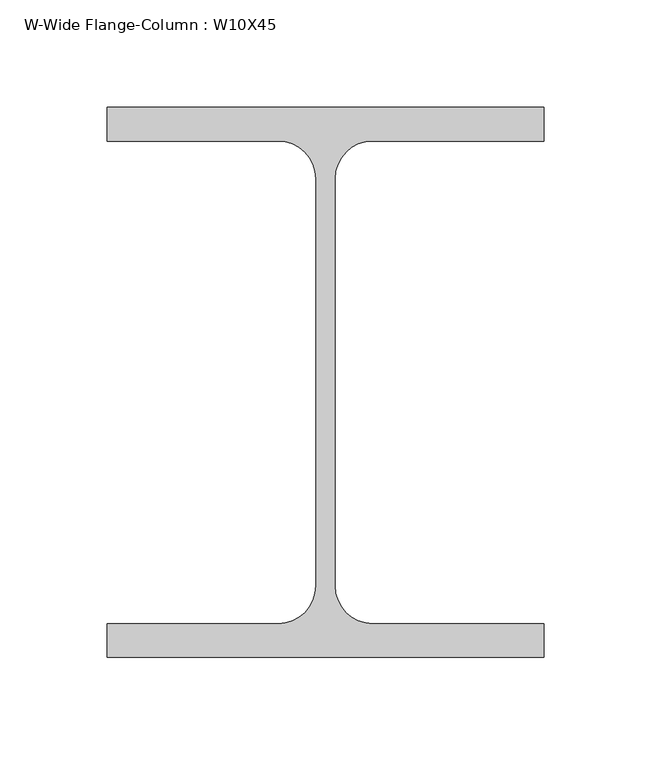
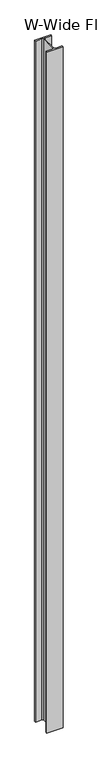
"""IFC4 building model written with IfcOpenShell, lengths in millimetres: column geometry, W-Wide Flange-Column : W10X45."""

from ifc_helpers import new_model, si_unit, point, frame, frame_2d, origin, place, context, project, spatial, polyline, circle_curve, trimmed, segment, composite_curve, outline, extrude, source, transform, mapped, element, save


def w_wide_flange_column_w10x45_58bd5f2d(model_context):
    return source(origin(), model_context, "Body", "SweptSolid", [
        extrude(outline(composite_curve([segment(polyline([(101.854, 128.27), (101.854, 112.522), (22.0345, 112.522)]), True, "CONTINUOUS"), segment(trimmed(circle_curve(frame_2d((22.0345, 94.9325)), 17.5895), [point((22.0345, 112.522))], [point((4.445, 94.9325))], True, "CARTESIAN"), True, "CONTINUOUS"), segment(polyline([(4.445, 94.9325), (4.445, -94.9325)]), True, "CONTINUOUS"), segment(trimmed(circle_curve(frame_2d((22.0345, -94.9325)), 17.5895), [point((4.445, -94.9325))], [point((22.0345, -112.522))], True, "CARTESIAN"), True, "CONTINUOUS"), segment(polyline([(22.0345, -112.522), (101.854, -112.522), (101.854, -128.27), (-101.854, -128.27), (-101.854, -112.522), (-22.0345, -112.522)]), True, "CONTINUOUS"), segment(trimmed(circle_curve(frame_2d((-22.0345, -94.9325)), 17.5895), [point((-22.0345, -112.522))], [point((-4.445, -94.9325))], True, "CARTESIAN"), True, "CONTINUOUS"), segment(polyline([(-4.445, -94.9325), (-4.445, 94.9325)]), True, "CONTINUOUS"), segment(trimmed(circle_curve(frame_2d((-22.0345, 94.9325)), 17.5895), [point((-4.445, 94.9325))], [point((-22.0345, 112.522))], True, "CARTESIAN"), True, "CONTINUOUS"), segment(polyline([(-22.0345, 112.522), (-101.854, 112.522), (-101.854, 128.27), (101.854, 128.27)]), True, "CONTINUOUS")], self_intersect=False)), frame((0.0, 0.0, 8655.05), z_axis=(0.0, 0.0, 1.0), x_axis=(1.0, 0.0, 0.0)), (0.0, 0.0, 1.0), 8972.55),
    ])


if __name__ == "__main__":
    model = new_model("IFC4")
    model_context = context("Model", 3, world=origin())
    ifc_project = project(units=[si_unit("LENGTHUNIT", "METRE", prefix="MILLI")], contexts=[model_context])
    site = spatial("IfcSite", under=ifc_project)
    building = spatial("IfcBuilding", under=site)
    placement = place(None, origin())
    w_wide_flange_column_w10x45_shape = w_wide_flange_column_w10x45_58bd5f2d(model_context)
    element("IfcColumn", 1, ObjectType="W-Wide Flange-Column : W10X45", at=placement, inside=building, context=model_context, shape_type="MappedRepresentation", body=[
        mapped(w_wide_flange_column_w10x45_shape, transform((0.0, 0.0, 0.0), x_axis=(1.0, 0.0, 0.0), y_axis=(0.0, 1.0, 0.0), z_axis=(0.0, 0.0, 1.0))),
    ])
    save(model, "model.ifc")

# Revit data of these elements
# Type "W-Wide Flange-Column : W10X45"
#   Assembly Code = "B10"
#   W = 45
#   bf = 0' - 8.02"
#   d = 0' - 10.1"
#   k = 0' - 1 5/16"
#   kr = 0' - 0.6925"
#   tf = 0' - 0.62"
#   tw = 0' - 0.35"
#   A = 0.0923611 SF
#   Structural Material [instance default] = Steel ASTM A992
# Element 1 (IfcColumn, "W-Wide Flange-Column : W10X45")
#   Materials on its faces: "Steel ASTM A992"
# Materials
#   "Steel ASTM A992": class "Metal", colour RGB 199 199 199, transparency 0, Description = "Structural steel 50ksi", Cost = 0
